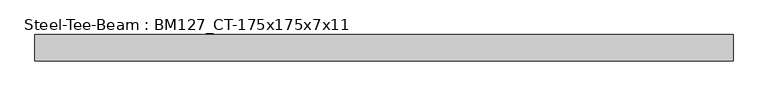
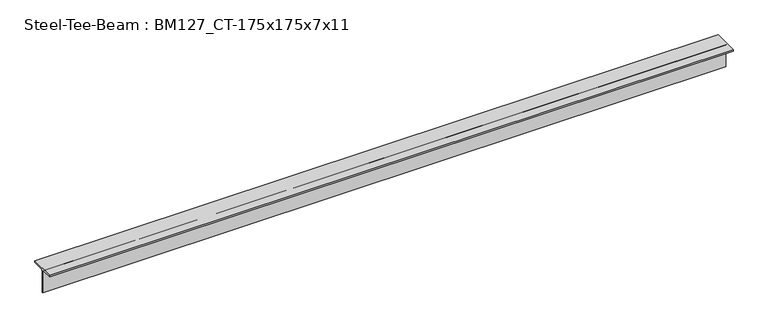
"""IFC4 building model written with IfcOpenShell, lengths in millimetres: beam geometry, Steel-Tee-Beam : BM127_CT-175x175x7x11."""

from ifc_helpers import new_model, si_unit, point, frame, frame_2d, origin, place, context, project, spatial, polyline, circle_curve, trimmed, segment, composite_curve, outline, extrude, source, transform, mapped, element, save


def steel_tee_beam_bm127_ct_175x175x7x11_9f293f4f(model_context):
    return source(origin(), model_context, "Body", "SweptSolid", [
        extrude(outline(composite_curve([segment(polyline([(-87.5, 87.5), (87.5, 87.5), (87.5, 76.5), (17.5, 76.5)]), True, "CONTINUOUS"), segment(trimmed(circle_curve(frame_2d((17.5, 62.5)), 14.0), [point((17.5, 76.5))], [point((3.5, 62.5))], True, "CARTESIAN"), True, "CONTINUOUS"), segment(polyline([(3.5, 62.5), (3.5, -87.5), (-3.5, -87.5), (-3.5, 62.5)]), True, "CONTINUOUS"), segment(trimmed(circle_curve(frame_2d((-17.5, 62.5)), 14.0), [point((-3.5, 62.5))], [point((-17.5, 76.5))], True, "CARTESIAN"), True, "CONTINUOUS"), segment(polyline([(-17.5, 76.5), (-87.5, 76.5), (-87.5, 87.5)]), True, "CONTINUOUS")], self_intersect=False)), frame((-2276.3489916, 0.0, 0.0), z_axis=(1.0, 0.0, 0.0), x_axis=(0.0, 1.0, 0.0)), (0.0, 0.0, 1.0), 4641.606963),
    ])


if __name__ == "__main__":
    model = new_model("IFC4")
    model_context = context("Model", 3, world=origin())
    ifc_project = project(units=[si_unit("LENGTHUNIT", "METRE", prefix="MILLI")], contexts=[model_context])
    site = spatial("IfcSite", under=ifc_project)
    building = spatial("IfcBuilding", under=site)
    placement = place(None, origin())
    steel_tee_beam_bm127_ct_175x175x7x11_shape = steel_tee_beam_bm127_ct_175x175x7x11_9f293f4f(model_context)
    element("IfcBeam", 1, ObjectType="Steel-Tee-Beam : BM127_CT-175x175x7x11", at=placement, inside=building, context=model_context, shape_type="MappedRepresentation", body=[
        mapped(steel_tee_beam_bm127_ct_175x175x7x11_shape, transform((0.0, 0.0, 0.0), x_axis=(1.0, 0.0, 0.0), y_axis=(0.0, 1.0, 0.0), z_axis=(0.0, 0.0, 1.0))),
    ])
    save(model, "model.ifc")

# Revit data of these elements
# Type "Steel-Tee-Beam : BM127_CT-175x175x7x11"
#   Section Area = 31.57 cm²
#   Mass per Unit Length = 24.80 kg/m
#   Length [instance default] = 1524 mm
#   bf = 175 mm
#   d = 175 mm
#   k = 25 mm
#   kr = 14 mm
#   tf = 11 mm
#   tw = 7 mm
#   hec_material4 [instance default] = none
#   hec_material3 [instance default] = none
#   hec_material2 [instance default] = none
#   hec_material1 [instance default] = none
#   Structural Material [instance default] = Steel, 45-345
#   Assembly Code = ""
# Element 1 (IfcBeam, "Steel-Tee-Beam : BM127_CT-175x175x7x11")
#   hec_material3 = F01AC000-00002_Building/Shelter Fire Proofing Work_Intumescent Coating Type_1 hr. rating (UL 1709))
#   hec_material1 = S03AA029-00001_Main Steel Structure Erection Work_Shelter/Building_Light Steel
#   Structural Material = S01AA003-00001_Main Steel Structure Fabrication Work_Shelter/Building_Light Steel - Standard
#   Materials on its faces: "S01AA003-00001_Main Steel Structure Fabrication Work_Shelter/Building_Light Steel - Standard"
# Materials
#   "Steel, 45-345": class "Metal", colour RGB 189 187 185, transparency 0, Description = "Steel 345 MPa", Cost = 0
#   "S01AA003-00001_Main Steel Structure Fabrication Work_Shelter/Building_Light Steel - Standard": class "Metal", colour RGB 120 120 120, transparency 0, Comments = "(30KG/M>Weight)", Description = "Structural steel 50ksi", W00) Work Master Code = "S01AA003-00001", W01) Work Master_Lv1 = "Main Steel Structure Fabrication Work", W02) Work Master_Lv2 = "Shelter/Building", W03) Work Master_Spec.1 = "Light Steel - Standard (30KG/M>Weight)", Cost = 0
#   "F01AC000-00002_Building/Shelter Fire Proofing Work_Intumescent Coating Type_1 hr. rating (UL 1709))": class "Metal", colour RGB 255 128 128, transparency 0, Description = "Paint finished steel", W00) Work Master Code = "F01AC000-00002", W01) Work Master_Lv1 = "Building/Shelter Fire Proofing Work", W02) Work Master_Lv2 = "Intumescent Coating Type", W03) Work Master_Spec.1 = "1 hr. rating (UL 1709)", Cost = 0
#   "S03AA029-00001_Main Steel Structure Erection Work_Shelter/Building_Light Steel": class "Metal", colour RGB 120 120 120, transparency 0, Comments = "(30KG/M>Weight)", Description = "Structural steel 50ksi", W00) Work Master Code = "S03AA029-00001", W01) Work Master_Lv1 = "Main Steel Structure Erection Work", W02) Work Master_Lv2 = "Shelter/Building", W03) Work Master_Spec.1 = "Light Steel (30KG/M>Weight)", Cost = 0
